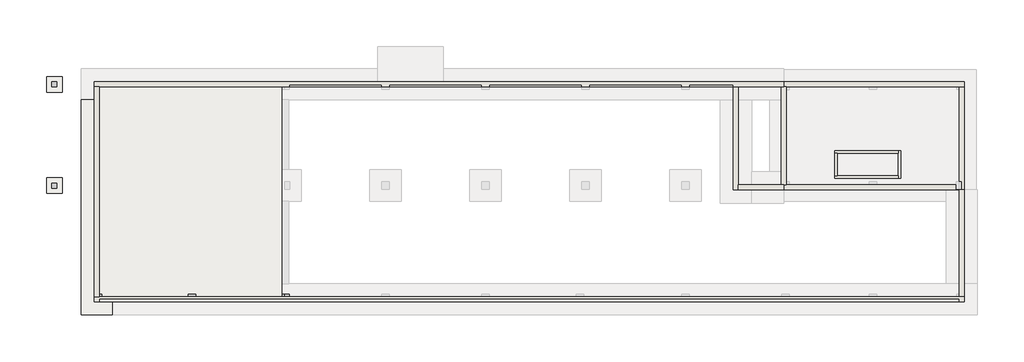
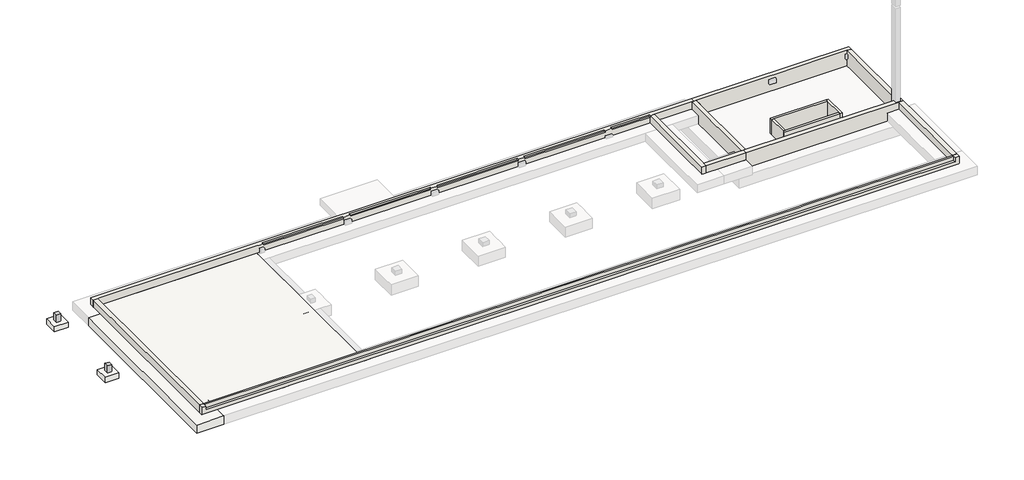
# Not in any storey, part 1 of 2: 14 walls, 5 columns, 3 slabs, 2 beams, 1 footing.
# Revit data of these elements (continued)
# Type "H_SF_AR_S18_Wall FDN_T800" (continued)
#   H_WM Code_6 = "A01ZZ001-00012 |  | M3 | Earth Work | - | Excavation | Soil, Mech. |  | Manual Excavation Above GWL |  |  |  | A01ZZ001-00012 Earth Work - Excavation Soil, Mech.      Manual Excavation Above GWL  | Above GWL"
#   H_WM Code_7 = "A01ZZ001-00013 |  | M3 | Earth Work | - | Excavation | Soil, Mech. |  | Manual Excavation Below GWL |  |  |  | A01ZZ001-00013 Earth Work - Excavation Soil, Mech.      Manual Excavation Below GWL  | Below GWL"
#   H_WM Code_8 = "A01ZZ003-00001 |  | M3 | Earth Work | - | Backfill | Re-use, Soil |  |  |  | Compaction=(  )% |  | A01ZZ003-00001 Earth Work - Backfill Re-use, Soil        | Compaction=( 95 )%"
#   H_WM Code_9 = "A01ZZ004-00001 |  | M3 | Earth Work | - | Disposal | Soil |  |  |  | Disposal Distance=Appx. (  )km from Site |  | A01ZZ004-00001 Earth Work - Disposal Soil        | Disposal Distance=Appx. (20 )km from Site"
#   H_WM Code_10 = "A03AH056-00001 |  | M2 | Concrete Work | Concrete Protective Coating (U/G) | Bitumen/Bituminous/Asphalt Coating |  |  | A03AH056-00001 Concrete Work Concrete Protective Coating (U/G) Bitumen/Bituminous/Asphalt Coating         | *기초바닥 Protection 은 Lean에 적용"
#   H_Rebar ratio = 0.3
# Type "H_FL_AR_S17_RC Slab T150_B1S1"
#   Keynote = ""
#   Type Comments = "CV-AG"
#   Description = ""
#   Type Mark = "B1S1"
#   H_Q'ty Cal Type Tag = "FL-Q1"
#   H_WM Code_1 = "A03AF032-00022 |  | M3 | Concrete Work | Superstructure Work | Structural Concrete | Cement Type-1 | 25MPa ≤ F'c (Cylinder Strength) < 30MPa |  |  |  |  | A03AF032-00022 Concrete Work Superstructure Work Structural Concrete  Cement Type-1 25MPa ≤ F'c (Cylinder Strength) < 30MPa      | ASTM C150 Type I or Type IA \nF'c (Cylinder Strength) = 28MPa"
#   H_WM Code_2 = "A03AF037-00003 |  | TON | Concrete Work | Superstructure Work | Rebar Work | Deformed Bar (Non-Coat.) | 300MPa<Fy≤400MPa |  |  |  |  | A03AF037-00003 Concrete Work Superstructure Work Rebar Work Deformed Bar (Non-Coat.)  300MPa<Fy≤400MPa      | KS D3504 SD400 (Fy=400MPa)"
#   H_WM Code_3 = "A03AF036-00001 |  | M2 | Concrete Work | Superstructure Work | Form Work (1 time in use) | Flat Form | Dressed Lumber, Plywood or Steel Form(Wood Planks are not Allowed) incl. Chamfer |  |  |  | A03AF036-00001 Concrete Work Superstructure Work Form Work (1 time in use) Flat Form     Dressed Lumber, Plywood or Steel Form(Wood Planks are not Allowed) incl. Chamfer   |"
#   H_WM Code_4 = "A04AS173-00001 |  | M2 | Finishing Work | Exterior/Interior Finish Work | Steel Trowel Finish |  |  |  |  | A04AS173-00001 Finishing Work Exterior/Interior Finish Work Steel Trowel Finish         |"
#   H_Rebar ratio = 0.1
#   Function = 1
#   Layers, outside or top first: 150 mm "00_Concrete_Reinf. Conc." (function 1)
# Type "Foundation Rectangular (Non-Pile) : H_SF_AR_S18_W1250xL1250xT500_Bitumen_F2"
#   Type Comments = "UG"
#   Type Mark = "F2"
#   H_Q'ty Cal Type Tag = "SB-Q1"
#   H_WM Code_1 = "A03AF032-00022 |  | M3 | Concrete Work | Superstructure Work | Structural Concrete | Cement Type-1 | 25MPa ≤ F'c (Cylinder Strength) < 30MPa |  |  |  |  | A03AF032-00022 Concrete Work Superstructure Work Structural Concrete  Cement Type-1 25MPa ≤ F'c (Cylinder Strength) < 30MPa      |  F'c (Cylinder Strength) = 24MPa"
#   H_WM Code_2 = "A03AD037-00002 |  | TON | Concrete Work | Substructure Work | Rebar Work | Deformed Bar (Non-Coat.) | 400MPa<Fy≤470MPa |  |  |  |  | A03AD037-00002 Concrete Work Substructure Work Rebar Work Deformed Bar (Non-Coat.)  400MPa<Fy≤470MPa      | ASTM A615 GRADE 60 (Fy=420MPa)"
#   H_WM Code_3 = "A03AF036-00001 |  | M2 | Concrete Work | Superstructure Work | Form Work (1 time in use) | Flat Form | Dressed Lumber, Plywood or Steel Form(Wood Planks are not Allowed) incl. Chamfer |  |  |  | A03AF036-00001 Concrete Work Superstructure Work Form Work (1 time in use) Flat Form     Dressed Lumber, Plywood or Steel Form(Wood Planks are not Allowed) incl. Chamfer   |"
#   Top bar = "D25@300"
#   Description = "UG Shallow Foundation"
#   Bottom bar = "D20@300"
#   Width = 1250 mm
#   Length = 1250 mm
#   Foundation Thickness = 500 mm
#   Structural Material [instance default] = none
#   Assembly Code = ""
# Type "H_WA_AR_B02_Ext Wall_RC T400_UG_Bitumen 2"
#   Type Comments = "CV-UG"
#   Type Mark = "W1A"
#   H_Q'ty Cal Type Tag = "WA-Q1"
#   H_WM Code_1 = "A03AF032-00022 |  | M3 | Concrete Work | Superstructure Work | Structural Concrete | Cement Type-1 | 25MPa ≤ F'c (Cylinder Strength) < 30MPa |  |  |  |  | A03AF032-00022 Concrete Work Superstructure Work Structural Concrete  Cement Type-1 25MPa ≤ F'c (Cylinder Strength) < 30MPa      | ASTM C150 Type I or Type IA \nF'c (Cylinder Strength) = 28MPa"
#   H_WM Code_2 = "A03AD037-00002 |  | TON | Concrete Work | Substructure Work | Rebar Work | Deformed Bar (Non-Coat.) | 400MPa<Fy≤470MPa |  |  |  |  | A03AD037-00002 Concrete Work Substructure Work Rebar Work Deformed Bar (Non-Coat.)  400MPa<Fy≤470MPa      | ASTM A615 GRADE 60 (Fy=420MPa)"
#   H_WM Code_3 = "A03AD036-00001 |  | M2 | Concrete Work | Substructure Work | Form Work (1 time in use) | Flat Form | Dressed Lumber, Plywood or Steel Form(Wood Planks are not Allowed) incl. Chamfer |  |  |  | A03AD036-00001 Concrete Work Substructure Work Form Work (1 time in use) Flat Form     Dressed Lumber, Plywood or Steel Form(Wood Planks are not Allowed) incl. Chamfer   |"
#   H_WM Code_4 = "A04AL076-00008 |  | M2 | Finishing Work | Masonry Work | Insulation | Glass Wool (Fiberglass) | Minimum Density of 50 kg/m3 | 100mm≤THK | THK=(  )mm |  | A04AL076-00008 Finishing Work Masonry Work Insulation Glass Wool (Fiberglass)     Minimum Density of 50 kg/m3  100mm≤THK | inside insulation"
#   H_WM Code_5 = "A04AS177-00004 |  | M2 | Finishing Work | Exterior/Interior Finish Work | Gypsumboard Partition Wall (Fixed Type) | Fire Protective Rating: N/A, 2-Layer Gypsum Boards to One Side | w/o Insulation | Including Supporting Frame(Stud) & Accessories | 1-Layer Gypsumboard THK=9.5mm |  |  | A04AS177-00004 Finishing Work Exterior/Interior Finish Work Gypsumboard Partition Wall (Fixed Type) Fire Protective Rating: N/A, 2-Layer Gypsum Boards to One Side   w/o Insulation  Including Supporting Frame(Stud) & Accessories  1-Layer Gypsumboard THK=9.5mm | gypsum board"
#   H_Rebar ratio = 0.12
#   Layers, outside or top first: 400 mm "00_Concrete_Reinf. Conc." (function 1)
# Type "H_WA_AR_B02_Ext Wall_RC T400_UG_Bitumen_W1A"
#   Type Comments = "CV-UG"
#   Type Mark = "W1A"
#   H_Q'ty Cal Type Tag = "WA-Q1"
#   H_WM Code_1 = "A03AD032-00025 |  | M3 | Concrete Work | Substructure Work | Structural Concrete | Cement Type-1 | 20MPa ≤ F'c (Cylinder Strength) < 25MPa |  |  |  |  | A03AD032-00025 Concrete Work Substructure Work Structural Concrete  Cement Type-1 20MPa ≤ F'c (Cylinder Strength) < 25MPa      | ASTM C150 Type I or Type IA \nF'c (Cylinder Strength) = 24MPa"
#   H_WM Code_2 = "A03AD037-00002 |  | TON | Concrete Work | Substructure Work | Rebar Work | Deformed Bar (Non-Coat.) | 400MPa<Fy≤470MPa |  |  |  |  | A03AD037-00002 Concrete Work Substructure Work Rebar Work Deformed Bar (Non-Coat.)  400MPa<Fy≤470MPa      | ASTM A615 GRADE 60 (Fy=420MPa)"
#   H_WM Code_3 = "A03AD036-00001 |  | M2 | Concrete Work | Substructure Work | Form Work (1 time in use) | Flat Form | Dressed Lumber, Plywood or Steel Form(Wood Planks are not Allowed) incl. Chamfer |  |  |  | A03AD036-00001 Concrete Work Substructure Work Form Work (1 time in use) Flat Form     Dressed Lumber, Plywood or Steel Form(Wood Planks are not Allowed) incl. Chamfer   |"
#   H_Rebar ratio = 0.12
#   Layers, outside or top first: 400 mm "00_Concrete_Reinf. Conc." (function 1)
# Type "H_WA_AR_B02_Int Wall_RC_Trench"
#   Type Comments = "CV-UG"
#   Type Mark = "trench"
#   H_Q'ty Cal Type Tag = "WA-Q1"
#   H_WM Code_1 = "A04AS177-00019 |  | M2 | Finishing Work | Exterior/Interior Finish Work | Gypsumboard Partition Wall (Fixed Type) | Fire Protective Rating: N/A, 2-Layer Gypsum Boards to Both Sides | Glass Wool (Fiberglass) | Including Supporting Frame(Stud) & Accessories | 1-Layer Gypsumboard THK=9.5mm | Insulation THK=(  )mm |  | A04AS177-00019 Finishing Work Exterior/Interior Finish Work Gypsumboard Partition Wall (Fixed Type) Fire Protective Rating: N/A, 2-Layer Gypsum Boards to Both Sides   Glass Wool (Fiberglass)  Including Supporting Frame(Stud) & Accessories  1-Layer Gypsumboard THK=9.5mm |"
#   H_WM Code_2 = "A04AL069-00002 |  | M2 | Finishing Work | Masonry Work | Reinforced Concrete Block | w/ All Reinf.(Lath, Steel Tie, Anchor Bar, Mortar, ETC.), Filler, Sealant, Lintel/Sill for Opening, ETC. | 100mm<THK≤200mm | THK=(  )mm |  | A04AL069-00002 Finishing Work Masonry Work Reinforced Concrete Block      w/ All Reinf.(Lath, Steel Tie, Anchor Bar, Mortar, ETC.), Filler, Sealant, Lintel/Sill for Opening, ETC.  100mm<THK≤200mm | THK=( 150)mm"
#   H_Rebar ratio = 0.12
#   Layers, outside or top first: 200 mm "00_Concrete_Reinf. Conc." (function 1)
# Element 1 (IfcBeam, "RC Beam_Rectangular : H_SB_AR_S16_TG_B500xH700_FB1")
#   Comments = ""
#   hec_material3 = none
#   hec_material2 = none
#   hec_material1 = none
#   Structural Material = 00_Concrete_Reinf. Conc.
#   Phase Created = New Construction
#   Materials on its faces: "00_Concrete_Reinf. Conc."
# Element 2 (IfcBeam, "RC Beam_Rectangular : H_SB_AR_S16_TG_B500xH700_FG1")
#   Comments = ""
#   hec_material3 = none
#   hec_material2 = none
#   hec_material1 = none
#   Structural Material = 00_Concrete_Reinf. Conc.
#   Phase Created = New Construction
#   Materials on its faces: "00_Concrete_Reinf. Conc."
# Elements 3, 4, 5 (IfcColumn, "RC_Column_Rectangular : H_SC_AR_S15_UG_W600xL600_C2")
#   Comments = ""
#   hec_material3 = none
#   hec_material2 = none
#   hec_material1 = none
#   Structural Material = 00_Concrete_Reinf. Conc.
#   Phase Created = New Construction
#   Materials on its faces: "00_Concrete_Reinf. Conc."
# Elements 6, 7 (IfcColumn, "RC_Column_Rectangular : H_SC_AR_S15_UG_W400xL400_C3")
#   Comments = ""
#   hec_material3 = none
#   hec_material2 = none
#   hec_material1 = none
#   Structural Material = 00_Concrete_Reinf. Conc.
#   Phase Created = New Construction
#   Materials on its faces: "00_Concrete_Reinf. Conc."
# Element 8 (IfcFooting, "H_SF_AR_S18_Wall FDN_T800")
#   Comments = ""
#   Phase Created = New Construction
#   Materials on its faces: "00_Concrete_Reinf. Conc."
# Element 9 (IfcSlab, "H_FL_AR_S17_RC Slab T150_B1S1")
#   Comments = ""
#   TMP_Element Name = "SS2"
#   Height Offset From Level = 800 mm
#   built-in parameter 1001954 = 1
#   Phase Created = New Construction
#   Materials on its faces: "00_Concrete_Reinf. Conc."
# Elements 10, 11 (IfcSlab, "Foundation Rectangular (Non-Pile) : H_SF_AR_S18_W1250xL1250xT500_Bitumen_F2")
#   Comments = ""
#   Structural Material = 00_Concrete_Reinf. Conc.
#   Phase Created = New Construction
#   Materials on its faces: "00_Concrete_Reinf. Conc."
# Elements 12, 13, 14, 15, 16, 17 (IfcWall, "H_WA_AR_B02_Ext Wall_RC T400_UG_Bitumen 2")
#   Comments = ""
#   built-in parameter 1001111 = 800 mm
#   Top Offset = 0 mm
#   Base Offset = 800 mm
#   wall height = 700 mm
#   Phase Created = New Construction
#   Base Constraint = BOF
#   Top Constraint = TOC
#   Materials on its faces: "00_Concrete_Reinf. Conc."
# Elements 18, 19, 20, 21 (IfcWall, "H_WA_AR_B02_Ext Wall_RC T400_UG_Bitumen_W1A")
#   Comments = ""
#   Top Offset = 0 mm
#   Base Offset = 0 mm
#   wall height = 1500 mm
#   Phase Created = New Construction
#   Base Constraint = BOF
#   Top Constraint = TOC
#   Materials on its faces: "00_Concrete_Reinf. Conc."
# Elements 22, 23, 24, 25 (IfcWall, "H_WA_AR_B02_Int Wall_RC_Trench")
#   Comments = ""
#   Top Offset = 0 mm
#   Base Offset = 0 mm
#   wall height = 1500 mm
#   Phase Created = New Construction
#   Base Constraint = BOF
#   Top Constraint = TOC
#   Materials on its faces: "00_Concrete_Reinf. Conc."
# Materials
#   "00_Concrete_Reinf. Conc.": class "Concrete", colour RGB 176 176 176, transparency 0, Description = "Reinf. Conc.", Cost = 0, Image = Concrete.Cast-In-Place.Flat.Polished.Grey.jpg
